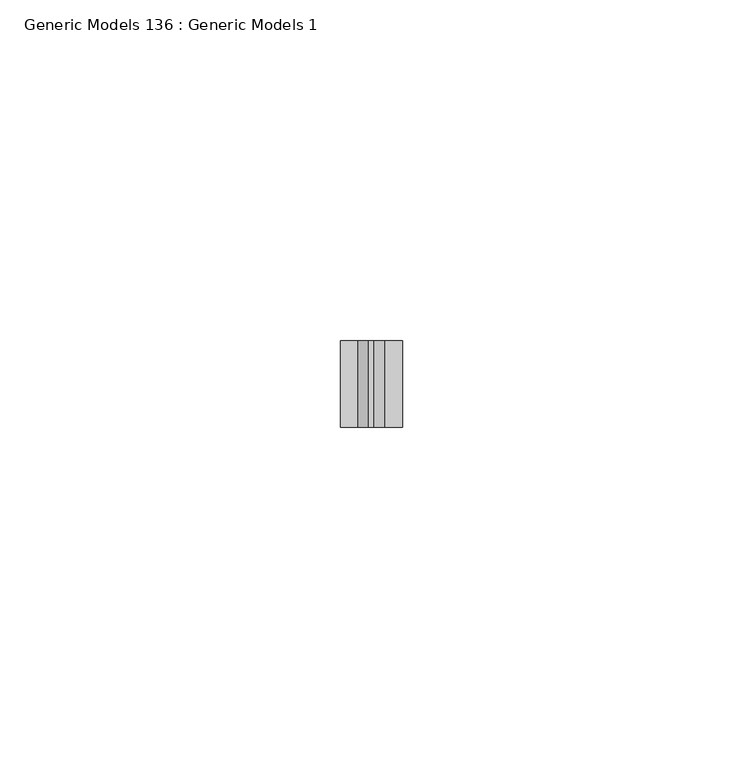
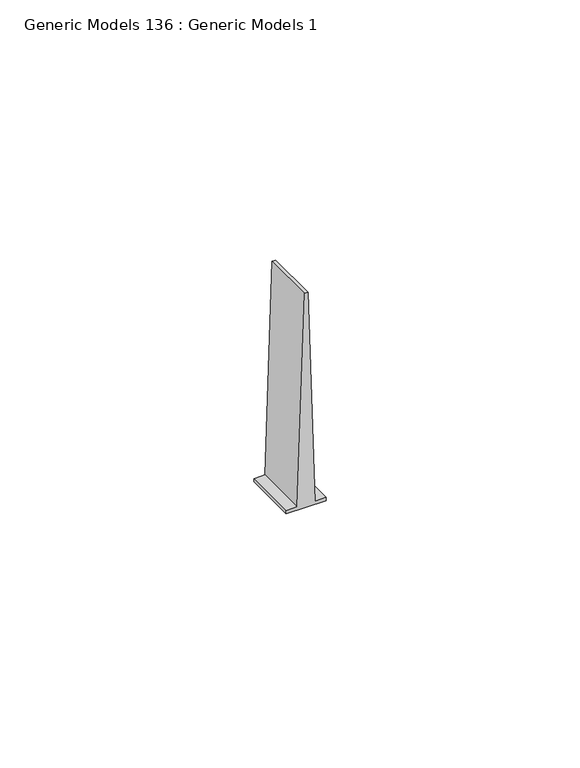
"""IFC4 building model written with IfcOpenShell, lengths in millimetres: proxy geometry, Generic Models 136 : Generic Models 1."""

from ifc_helpers import new_model, si_unit, frame, origin, place, context, project, spatial, polyline, outline, extrude, source, transform, mapped, element, save


def generic_models_136_generic_models_1_7576d418(model_context):
    return source(origin(), model_context, "Body", "SweptSolid", [
        extrude(outline(polyline([(2229.092683, 46885.2894531), (2229.092683, 46894.3826531), (2229.886433, 46894.3826531), (2229.886433, 46891.8327895), (2280.686433, 46890.2354003), (2280.686433, 46889.4367058), (2229.886433, 46887.8393167), (2229.886433, 46885.2894531), (2229.092683, 46885.2894531)])), frame((0.0, 565.15, 0.0), z_axis=(0.0, 1.0, 0.0), x_axis=(0.0, 0.0, 1.0)), (0.0, 0.0, 1.0), 12.7),
    ])


if __name__ == "__main__":
    model = new_model("IFC4")
    model_context = context("Model", 3, world=origin())
    ifc_project = project(units=[si_unit("LENGTHUNIT", "METRE", prefix="MILLI")], contexts=[model_context])
    site = spatial("IfcSite", under=ifc_project)
    building = spatial("IfcBuilding", under=site)
    placement = place(None, origin())
    generic_models_136_generic_models_1_shape = generic_models_136_generic_models_1_7576d418(model_context)
    element("IfcBuildingElementProxy", 1, Name="Generic Models 136 : Generic Models 1", ObjectType="Generic Models 136 : Generic Models 1", at=placement, inside=building, context=model_context, shape_type="MappedRepresentation", body=[
        mapped(generic_models_136_generic_models_1_shape, transform((0.0, 0.0, 0.0), x_axis=(1.0, 0.0, 0.0), y_axis=(0.0, 1.0, 0.0), z_axis=(0.0, 0.0, 1.0))),
    ])
    save(model, "model.ifc")

# Revit data of these elements
# Element 1 (IfcBuildingElementProxy, "Generic Models 136 : Generic Models 1")
#   Materials on its faces: "METAL RUNNER CHANNEL; FASTEN @ 24\" O.C."
# Materials
#   "METAL RUNNER CHANNEL; FASTEN @ 24\" O.C.": class "Unassigned", colour RGB 210 209 208, transparency 0, Keynote = "M05121300.02", Cost = 0
